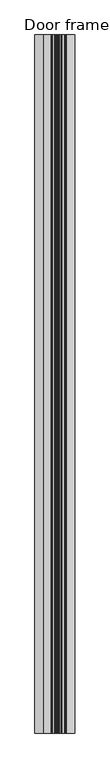
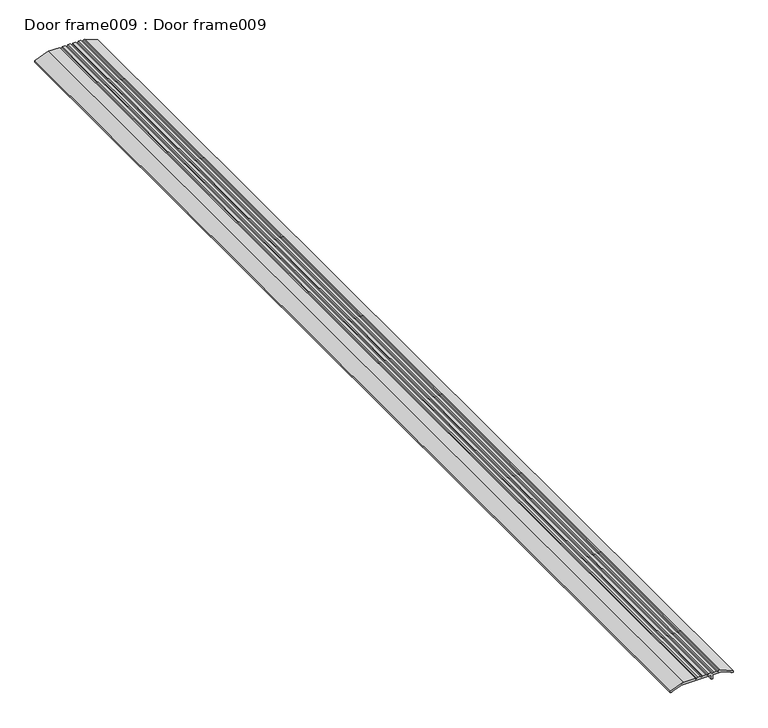
"""IFC4 building model written with IfcOpenShell, lengths in millimetres: proxy geometry, Door frame009 : Door frame009."""

import ifcopenshell
import ifcopenshell.guid

model = None  # the IFC model being written
_history = None  # IfcOwnerHistory: only IFC2X3 demands one
_inside = {}  # id of a spatial element -> (the spatial element, [elements in it])
_under = {}  # id of a project, library or spatial element -> (it, [spatial elements below it])
_declared = {}  # id of a project -> (the project, [libraries it declares])
_typed = {}  # id of a type object -> (the type object, [elements of that type])
_made_of = {}  # id of a material, layer set ... -> (it, [elements and type objects made of it])


def new_model(schema):
    """Start an empty IFC model of exactly this schema.

    Asked for "IFC4X3", IfcOpenShell would pick the latest addendum, in which some entities
    have other attributes; the version numbers below select the first issue.
    IFC2X3 requires an IfcOwnerHistory on every rooted entity: one is made here for all.
    """
    global model, _history
    if schema == "IFC4X3":
        model = ifcopenshell.file(schema_version=(4, 3, 0, 0))
    else:
        model = ifcopenshell.file(schema=schema)
    _inside.clear()
    _under.clear()
    _declared.clear()
    _typed.clear()
    _made_of.clear()
    _history = None
    if model.schema == "IFC2X3":
        org = make("IfcOrganization", Name="unknown")
        user = make(
            "IfcPersonAndOrganization",
            ThePerson=make("IfcPerson", FamilyName="unknown"),
            TheOrganization=org,
        )
        app = make(
            "IfcApplication",
            ApplicationDeveloper=org,
            Version="unknown",
            ApplicationFullName="unknown",
            ApplicationIdentifier="unknown",
        )
        _history = make(
            "IfcOwnerHistory",
            OwningUser=user,
            OwningApplication=app,
            ChangeAction="ADDED",
            CreationDate=0,
        )
    return model


def make(cls, **values):
    """One entity of the class cls with the attributes given. An attribute that is None is left unset."""
    return model.create_entity(
        cls, **{name: value for name, value in values.items() if value is not None}
    )


def rooted(cls, **values):
    """An entity with a GlobalId (a new one), such as an element, a storey or a relation."""
    return make(cls, GlobalId=ifcopenshell.guid.new(), OwnerHistory=_history, **values)


def si_unit(unit_type, name, prefix=None):
    """IfcSIUnit, for example si_unit("LENGTHUNIT", "METRE", prefix="MILLI")."""
    return make("IfcSIUnit", UnitType=unit_type, Prefix=prefix, Name=name)


def assignment(units):
    """IfcUnitAssignment: the units of a project."""
    return None if units is None else make("IfcUnitAssignment", Units=units)


def point(xyz):
    """IfcCartesianPoint."""
    return None if xyz is None else make("IfcCartesianPoint", Coordinates=xyz)


def direction(xyz):
    """IfcDirection."""
    return None if xyz is None else make("IfcDirection", DirectionRatios=xyz)


def frame(location, z_axis=None, x_axis=None):
    """IfcAxis2Placement3D, a coordinate frame: its origin and axes. An axis left out is left unset."""
    return make(
        "IfcAxis2Placement3D",
        Location=point(location),
        Axis=direction(z_axis),
        RefDirection=direction(x_axis),
    )


def origin():
    """The frame at (0, 0, 0) with its axes left unset."""
    return frame((0.0, 0.0, 0.0))


def place(relative_to, where):
    """IfcLocalPlacement: puts the frame where relative to a parent placement (None: the world)."""
    return make(
        "IfcLocalPlacement", PlacementRelTo=relative_to, RelativePlacement=where
    )


def context(
    kind, dimensions, precision=None, world=None, true_north=None, identifier=None
):
    """IfcGeometricRepresentationContext, for example the 3D "Model" context."""
    return make(
        "IfcGeometricRepresentationContext",
        ContextIdentifier=identifier,
        ContextType=kind,
        CoordinateSpaceDimension=dimensions,
        Precision=precision,
        WorldCoordinateSystem=world,
        TrueNorth=true_north,
    )


def project(units=None, contexts=None):
    """IfcProject with its units and contexts."""
    return rooted(
        "IfcProject",
        Name="project",
        RepresentationContexts=contexts,
        UnitsInContext=assignment(units),
    )


def spatial(cls, under=None, at=None, **own):
    """A site, building, storey or space (cls), placed at a placement, below another one or the project."""
    s = rooted(cls, ObjectPlacement=at, **own)
    if under is not None:
        _under.setdefault(under.id(), (under, []))[1].append(s)
    return s


def polyline(points):
    """IfcPolyline through the points."""
    return make("IfcPolyline", Points=[point(p) for p in points])


def outline(outer, holes=None, kind="AREA"):
    """IfcArbitraryClosedProfileDef: a profile drawn as a closed curve; with holes, ...WithVoids."""
    if holes is None:
        return make("IfcArbitraryClosedProfileDef", ProfileType=kind, OuterCurve=outer)
    return make(
        "IfcArbitraryProfileDefWithVoids",
        ProfileType=kind,
        OuterCurve=outer,
        InnerCurves=holes,
    )


def extrude(swept, where, along, depth):
    """IfcExtrudedAreaSolid: the profile swept, set in the frame where, extruded along a direction by depth."""
    return make(
        "IfcExtrudedAreaSolid",
        SweptArea=swept,
        Position=where,
        ExtrudedDirection=direction(along),
        Depth=depth,
    )


def shape(context_of_items, identifier, shape_type, items):
    """IfcShapeRepresentation: the items that make up one representation, for example the "Body"."""
    return make(
        "IfcShapeRepresentation",
        ContextOfItems=context_of_items,
        RepresentationIdentifier=identifier,
        RepresentationType=shape_type,
        Items=items,
    )


def source(mapping_origin, context_of_items, identifier, shape_type, items):
    """IfcRepresentationMap: a shape defined once, which mapped items show again and again."""
    return make(
        "IfcRepresentationMap",
        MappingOrigin=mapping_origin,
        MappedRepresentation=shape(context_of_items, identifier, shape_type, items),
    )


def transform(
    local_origin,
    x_axis=None,
    y_axis=None,
    z_axis=None,
    scale=None,
    scale2=None,
    scale3=None,
    uniform=True,
):
    """IfcCartesianTransformationOperator3D, or its non-uniform kind. x_axis, y_axis, z_axis: its Axis1, 2, 3."""
    if uniform:
        return make(
            "IfcCartesianTransformationOperator3D",
            Axis1=direction(x_axis),
            Axis2=direction(y_axis),
            LocalOrigin=point(local_origin),
            Scale=scale,
            Axis3=direction(z_axis),
        )
    return make(
        "IfcCartesianTransformationOperator3DnonUniform",
        Axis1=direction(x_axis),
        Axis2=direction(y_axis),
        LocalOrigin=point(local_origin),
        Scale=scale,
        Axis3=direction(z_axis),
        Scale2=scale2,
        Scale3=scale3,
    )


def mapped(mapping_source, mapping_target):
    """IfcMappedItem: shows the shape of a source again, moved by a transform."""
    return make(
        "IfcMappedItem", MappingSource=mapping_source, MappingTarget=mapping_target
    )


def made_of(thing, what):
    """Note that an element or type object is made of a material, layer set ...; save() writes the relation."""
    if what is not None:
        _made_of.setdefault(what.id(), (what, []))[1].append(thing)
    return thing


def element(
    cls,
    number,
    at=None,
    inside=None,
    cuts=None,
    type_object=None,
    material=None,
    context=None,
    identifier="Body",
    shape_type=None,
    held_by="IfcProductDefinitionShape",
    body=None,
    shapes=None,
    **own,
):
    """One element of the class cls, such as IfcWall. Its Tag is "e" and its number.

    at: its placement. inside: the storey or other place that contains it. cuts: it is an
    opening in that element (IfcRelVoidsElement). A single representation is given by context,
    identifier, shape_type and body (its items); several are given by shapes. held_by: the class
    of the entity that holds the representations. save() writes the other relations.
    """
    e = rooted(cls, Tag="e%d" % number, ObjectPlacement=at, **own)
    if body is not None:
        shapes = [shape(context, identifier, shape_type, body)]
    if shapes is not None:
        e.Representation = make(held_by, Representations=shapes)
    if inside is not None:
        _inside.setdefault(inside.id(), (inside, []))[1].append(e)
    if cuts is not None:
        rooted(
            "IfcRelVoidsElement", RelatingBuildingElement=cuts, RelatedOpeningElement=e
        )
    if type_object is not None:
        _typed.setdefault(type_object.id(), (type_object, []))[1].append(e)
    return made_of(e, material)


def aggregate(whole, parts):
    """IfcRelAggregates: a whole, such as a stair, and the parts it consists of."""
    return rooted("IfcRelAggregates", RelatingObject=whole, RelatedObjects=parts)


def save(model, path):
    """Write the relations noted so far, then the file.

    IfcRelAggregates (storeys below a building ...), IfcRelContainedInSpatialStructure (elements
    in a storey), IfcRelDefinesByType, IfcRelAssociatesMaterial and IfcRelDeclares: one each for
    every whole, place, type object, material and project.
    """
    for whole, parts in _under.values():
        aggregate(whole, parts)
    for where, things in _inside.values():
        rooted(
            "IfcRelContainedInSpatialStructure",
            RelatedElements=things,
            RelatingStructure=where,
        )
    for kind, things in _typed.values():
        rooted("IfcRelDefinesByType", RelatedObjects=things, RelatingType=kind)
    for what, things in _made_of.values():
        rooted("IfcRelAssociatesMaterial", RelatedObjects=things, RelatingMaterial=what)
    for by, libraries in _declared.values():
        rooted("IfcRelDeclares", RelatingContext=by, RelatedDefinitions=libraries)
    model.write(path)


def door_frame009_door_frame009_747449c1(model_context):
    return source(origin(), model_context, "Body", "SweptSolid", [
        extrude(outline(polyline([(36582.0975353, 15569.2471527), (36582.0975353, 15564.3576527), (36580.0353123, 15563.1670277), (36580.0353123, 15560.7857777), (36582.0975353, 15559.5951527), (36582.0975353, 15554.7056527), (36580.0353123, 15553.5150277), (36580.0353123, 15551.1337777), (36582.0975353, 15549.9431527), (36582.0975353, 15528.6904507), (36572.5243303, 15504.8264027), (36569.3983841, 15504.8264027), (36569.3983841, 15508.0014027), (36570.3770561, 15508.0014027), (36577.3350353, 15525.3462262), (36577.3350353, 15579.7549595), (36569.5937593, 15579.7549595), (36569.5937593, 15582.2978458), (36577.3350353, 15582.2978458), (36577.3350353, 15598.6065792), (36570.3770561, 15615.9514027), (36569.3983841, 15615.9514027), (36569.3983841, 15619.1264027), (36572.5243303, 15619.1264027), (36582.0975353, 15595.2623546), (36582.0975353, 15593.3136527), (36580.0353123, 15592.1230277), (36580.0353123, 15589.7417777), (36582.0975353, 15588.5511527), (36582.0975353, 15583.6616527), (36580.0353123, 15582.4710277), (36580.0353123, 15580.0897777), (36582.0975353, 15578.8991527), (36582.0975353, 15574.0096527), (36580.0353123, 15572.8190277), (36580.0353123, 15570.4377777), (36582.0975353, 15569.2471527)])), frame((0.0, -1052.8906567, 0.0), z_axis=(0.0, 1.0, 0.0), x_axis=(0.0, 0.0, 1.0)), (0.0, 0.0, 1.0), 1999.85),
    ])


if __name__ == "__main__":
    model = new_model("IFC4")
    model_context = context("Model", 3, world=origin())
    ifc_project = project(units=[si_unit("LENGTHUNIT", "METRE", prefix="MILLI")], contexts=[model_context])
    site = spatial("IfcSite", under=ifc_project)
    building = spatial("IfcBuilding", under=site)
    placement = place(None, origin())
    door_frame009_door_frame009_shape = door_frame009_door_frame009_747449c1(model_context)
    element("IfcBuildingElementProxy", 1, Name="Door frame009 : Door frame009", ObjectType="Door frame009 : Door frame009", at=placement, inside=building, context=model_context, shape_type="MappedRepresentation", body=[
        mapped(door_frame009_door_frame009_shape, transform((0.0, 0.0, 0.0), x_axis=(1.0, 0.0, 0.0), y_axis=(0.0, 1.0, 0.0), z_axis=(0.0, 0.0, 1.0))),
    ])
    save(model, "model.ifc")

# Revit data of these elements
# Type "Door frame009 : Door frame009"
#   NameOverride = "Door frame009"
# Element 1 (IfcBuildingElementProxy, "Door frame009 : Door frame009")
#   Materials on its faces: "ALUM. THRESHOLD"
# Materials
#   "ALUM. THRESHOLD": class "Metal", colour RGB 247 247 247, transparency 0, Description = "Aluminum 6061", Cost = 0
